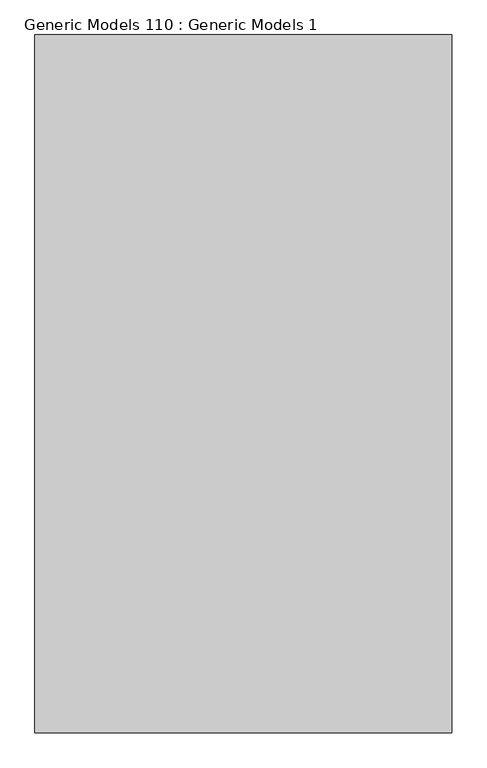
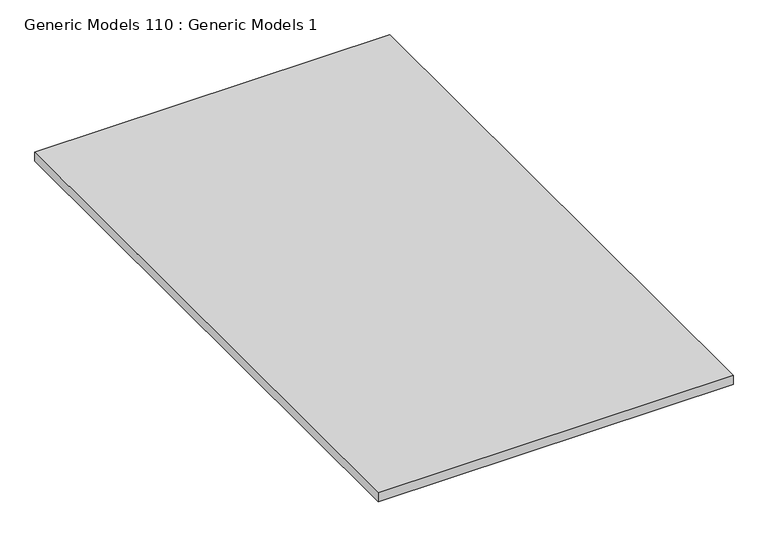
"""IFC4 building model written with IfcOpenShell, lengths in millimetres: proxy geometry, Generic Models 110 : Generic Models 1."""

from ifc_helpers import new_model, si_unit, frame, origin, place, context, project, spatial, polyline, outline, extrude, source, transform, mapped, element, save


def generic_models_110_generic_models_1_6bdce9b6(model_context):
    return source(origin(), model_context, "Body", "SweptSolid", [
        extrude(outline(polyline([(51642.1451407, 1219.2), (51642.1451407, 0.0), (50914.3, 0.0), (50914.3, 1219.2), (51642.1451407, 1219.2)])), frame((0.0, 0.0, 5508.228125), z_axis=(0.0, 0.0, 1.0), x_axis=(1.0, 0.0, 0.0)), (0.0, 0.0, 1.0), 19.05),
    ])


if __name__ == "__main__":
    model = new_model("IFC4")
    model_context = context("Model", 3, world=origin())
    ifc_project = project(units=[si_unit("LENGTHUNIT", "METRE", prefix="MILLI")], contexts=[model_context])
    site = spatial("IfcSite", under=ifc_project)
    building = spatial("IfcBuilding", under=site)
    placement = place(None, origin())
    generic_models_110_generic_models_1_shape = generic_models_110_generic_models_1_6bdce9b6(model_context)
    element("IfcBuildingElementProxy", 1, Name="Generic Models 110 : Generic Models 1", ObjectType="Generic Models 110 : Generic Models 1", at=placement, inside=building, context=model_context, shape_type="MappedRepresentation", body=[
        mapped(generic_models_110_generic_models_1_shape, transform((0.0, 0.0, 0.0), x_axis=(1.0, 0.0, 0.0), y_axis=(0.0, 1.0, 0.0), z_axis=(0.0, 0.0, 1.0))),
    ])
    save(model, "model.ifc")

# Revit data of these elements
# Element 1 (IfcBuildingElementProxy, "Generic Models 110 : Generic Models 1")
#   Materials on its faces: "3/4\" CDX PLYWOOD"
# Materials
#   "3/4\" CDX PLYWOOD": class "Unassigned", colour RGB 196 177 123, transparency 0, Cost = 0
